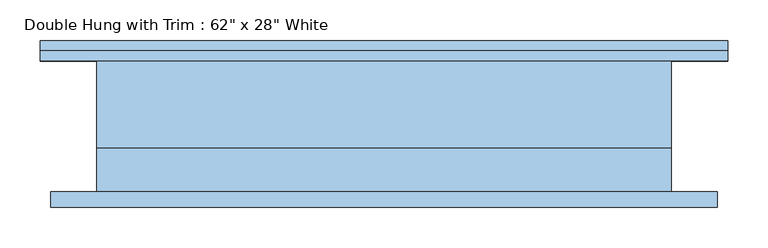
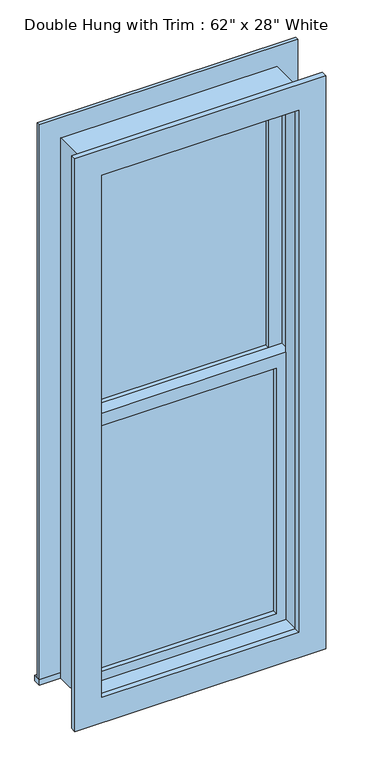
"""IFC4 building model written with IfcOpenShell, lengths in millimetres: window geometry."""

from ifc_helpers import new_model, si_unit, frame, origin, place, context, project, spatial, polyline, outline, extrude, source, transform, mapped, element, save


def window_6fcd84cf(model_context):
    return source(origin(), model_context, "Body", "SweptSolid", [
        extrude(outline(polyline([(-292.1, 1.5875), (292.1, 1.5875), (292.1, -11.1125), (-292.1, -11.1125), (-292.1, 1.5875)])), frame((0.0, 0.0, 977.9), z_axis=(0.0, 0.0, 1.0), x_axis=(1.0, 0.0, 0.0)), (0.0, 0.0, 1.0), 854.075),
        extrude(outline(polyline([(1876.425, -336.55), (933.45, -336.55), (933.45, 336.55), (1876.425, 336.55), (1876.425, -336.55)]), holes=[polyline([(1831.975, -292.1), (1831.975, 292.1), (977.9, 292.1), (977.9, -292.1), (1831.975, -292.1)])]), frame((0.0, -26.9875, 0.0), z_axis=(0.0, 1.0, 0.0), x_axis=(0.0, 0.0, 1.0)), (0.0, 0.0, 1.0), 44.45),
        extrude(outline(polyline([(-425.45, 106.3625), (425.45, 106.3625), (425.45, 80.9625), (-425.45, 80.9625), (-425.45, 106.3625)])), frame((0.0, 0.0, 914.4), z_axis=(0.0, 0.0, 1.0), x_axis=(1.0, 0.0, 0.0)), (0.0, 0.0, 1.0), 19.05),
        extrude(outline(polyline([(2774.95, -336.55), (2774.95, 336.55), (933.45, 336.55), (933.45, 425.45), (2863.85, 425.45), (2863.85, -425.45), (933.45, -425.45), (933.45, -336.55), (2774.95, -336.55)])), frame((0.0, 80.9625, 0.0), z_axis=(0.0, 1.0, 0.0), x_axis=(0.0, 0.0, 1.0)), (0.0, 0.0, 1.0), 12.7),
        extrude(outline(polyline([(2851.15, 412.75), (2851.15, -412.75), (857.25, -412.75), (857.25, 412.75), (2851.15, 412.75)]), holes=[polyline([(2762.25, 323.85), (946.15, 323.85), (946.15, -323.85), (2762.25, -323.85), (2762.25, 323.85)])]), frame((0.0, -100.0125, 0.0), z_axis=(0.0, 1.0, 0.0), x_axis=(0.0, 0.0, 1.0)), (0.0, 0.0, 1.0), 19.05),
        extrude(outline(polyline([(292.1, 33.3375), (-292.1, 33.3375), (-292.1, 46.0375), (292.1, 46.0375), (292.1, 33.3375)])), frame((0.0, 0.0, 1876.425), z_axis=(0.0, 0.0, 1.0), x_axis=(1.0, 0.0, 0.0)), (0.0, 0.0, 1.0), 854.075),
        extrude(outline(polyline([(2774.95, -336.55), (1831.975, -336.55), (1831.975, 336.55), (2774.95, 336.55), (2774.95, -336.55)]), holes=[polyline([(2730.5, -292.1), (2730.5, 292.1), (1876.425, 292.1), (1876.425, -292.1), (2730.5, -292.1)])]), frame((0.0, 17.4625, 0.0), z_axis=(0.0, 1.0, 0.0), x_axis=(0.0, 0.0, 1.0)), (0.0, 0.0, 1.0), 44.45),
        extrude(outline(polyline([(2794.0, -355.6), (914.4, -355.6), (914.4, 355.6), (2794.0, 355.6), (2794.0, -355.6)]), holes=[polyline([(2762.25, -323.85), (2762.25, 323.85), (946.15, 323.85), (946.15, -323.85), (2762.25, -323.85)])]), frame((0.0, -80.9625, 0.0), z_axis=(0.0, 1.0, 0.0), x_axis=(0.0, 0.0, 1.0)), (0.0, 0.0, 1.0), 53.975),
        extrude(outline(polyline([(2794.0, 355.6), (2794.0, -355.6), (914.4, -355.6), (914.4, 355.6), (2794.0, 355.6)]), holes=[polyline([(2774.95, 336.55), (933.45, 336.55), (933.45, -336.55), (2774.95, -336.55), (2774.95, 336.55)])]), frame((0.0, -26.9875, 0.0), z_axis=(0.0, 1.0, 0.0), x_axis=(0.0, 0.0, 1.0)), (0.0, 0.0, 1.0), 107.95),
    ])


if __name__ == "__main__":
    model = new_model("IFC4")
    model_context = context("Model", 3, world=origin())
    ifc_project = project(units=[si_unit("LENGTHUNIT", "METRE", prefix="MILLI")], contexts=[model_context])
    site = spatial("IfcSite", under=ifc_project)
    building = spatial("IfcBuilding", under=site)
    placement = place(None, origin())
    window_shape = window_6fcd84cf(model_context)
    element("IfcWindow", 1, ObjectType="Double Hung with Trim : 62\" x 28\" White", at=placement, inside=building, context=model_context, shape_type="MappedRepresentation", body=[
        mapped(window_shape, transform((0.0, 0.0, 0.0), x_axis=(1.0, 0.0, 0.0), y_axis=(0.0, 1.0, 0.0), z_axis=(0.0, 0.0, 1.0))),
    ])
    save(model, "model.ifc")

# Revit data of these elements
# Type "Double Hung with Trim : 62\" x 28\" White"
#   Type Mark = "79"
#   Construction Type Id = "GSP4R"
#   Assembly Code = "B2020100"
#   Analytic Construction = "1/8 in Pilkington single glazing"
#   Visual Light Transmittance = 0.9
#   Solar Heat Gain Coefficient = 0.78
#   Heat Transfer Coefficient (U) = 3.6886 W/(m²·K)
#   Height = 6' - 2"
#   Default Sill Height = 3' - 0"
#   Trim Projection - Ext. = 0' - 0 1/2"
#   Trim Projection - Int. = 0' - 0 3/4"
#   Trim Width - Exterior = 0' - 3 1/2"
#   Trim Width - Interior = 0' - 3 1/2"
#   Width = 2' - 4"
#   Window Inset = 0' - 0 3/4"
#   COBie.Type = no
#   Glass Pane Material = Glass
#   Sash Material = Sash - White
#   Trim Exterior Material = Trim - White
#   Trim Interior Material = Trim - White
#   Wall Closure = (empty or 0)
# Element 1 (IfcWindow, "Double Hung with Trim : 62\" x 28\" White")
#   Materials on its faces: "Sash - White", "Trim - White", "Glass"
# Materials
#   "Glass": class "Glass", colour RGB 0 128 192, transparency 0.75, Description = "Soda Lime Glass", Cost = 0
#   "Sash - White": class "Wood", colour RGB 255 255 255, transparency 0, Cost = 0
#   "Trim - White": class "Wood", colour RGB 255 255 255, transparency 0, Cost = 0
